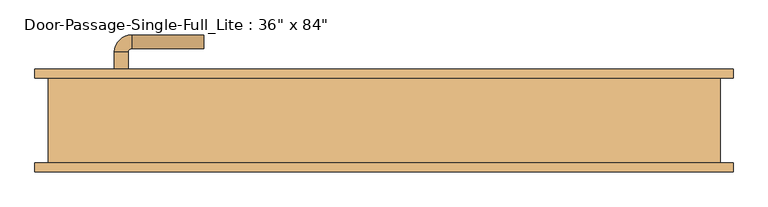
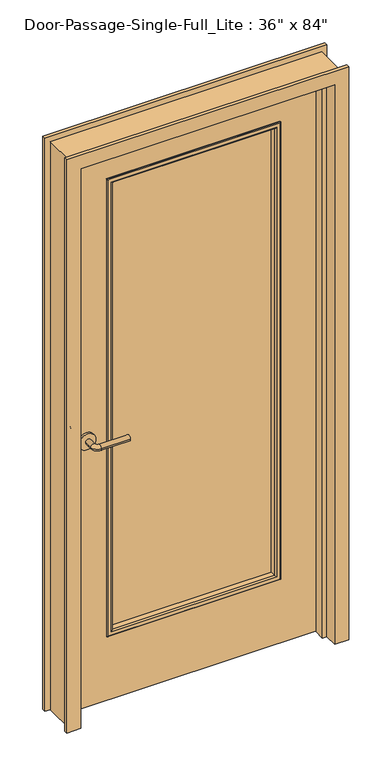
"""IFC4 building model written with IfcOpenShell, lengths in millimetres: door geometry."""

from ifc_helpers import new_model, si_unit, point, frame, frame_2d, origin, place, context, project, spatial, polyline, circle_curve, ellipse_curve, trimmed, segment, composite_curve, outline, extrude, faceted_brep, source, transform, mapped, element, save
from ifc_brep_helpers import plane_surface, cylinder_surface, revolved_surface, advanced_brep


def door_297712db(model_context):
    return source(origin(), model_context, "Body", "SolidModel", [
        advanced_brep(
        [(-392.190625, 15.8125, 1016.0), (-372.190625, 15.8125, 1016.0), (-372.190625, -14.1875, 1016.0), (-392.190625, -14.1875, 1016.0), (-367.190625, -19.1875, 1016.0), (-367.190625, -39.1875, 1016.0), (-262.190625, -39.1875, 1016.0), (-262.190625, -19.1875, 1016.0)],
        [
            (0, 1, circle_curve(frame((-382.190625, 15.8125, 1016.0), z_axis=(0.0, 1.0, 0.0), x_axis=(1.0, 0.0, 0.0)), 10.0)),
            (1, 0, circle_curve(frame((-382.190625, 15.8125, 1016.0), z_axis=(0.0, 1.0, 0.0), x_axis=(1.0, 0.0, 0.0)), 10.0)),
            (1, 2),
            (2, 3, circle_curve(frame((-382.190625, -14.1875, 1016.0), z_axis=(0.0, 1.0, 0.0), x_axis=(1.0, 0.0, 0.0)), 10.0)),
            (3, 0),
            (3, 2, circle_curve(frame((-382.190625, -14.1875, 1016.0), z_axis=(0.0, 1.0, 0.0), x_axis=(1.0, 0.0, 0.0)), 10.0)),
            (4, 5, circle_curve(frame((-367.190625, -29.1875, 1016.0), z_axis=(-1.0, 0.0, 0.0), x_axis=(0.0, 1.0, 0.0)), 10.0)),
            (5, 3, circle_curve(frame((-367.190625, -14.1875, 1016.0), z_axis=(0.0, 0.0, -1.0), x_axis=(-1.0, 0.0, 0.0)), 25.0)),
            (2, 4, circle_curve(frame((-367.190625, -14.1875, 1016.0), z_axis=(0.0, 0.0, 1.0), x_axis=(-1.0, 0.0, 0.0)), 5.0)),
            (5, 4, circle_curve(frame((-367.190625, -29.1875, 1016.0), z_axis=(-1.0, 0.0, 0.0), x_axis=(0.0, 1.0, 0.0)), 10.0)),
            (6, 7, circle_curve(frame((-262.190625, -29.1875, 1016.0), z_axis=(1.0, 0.0, 0.0), x_axis=(0.0, 1.0, 0.0)), 10.0)),
            (7, 6, circle_curve(frame((-262.190625, -29.1875, 1016.0), z_axis=(1.0, 0.0, 0.0), x_axis=(0.0, 1.0, 0.0)), 10.0)),
            (4, 7),
            (6, 5),
        ],
        [
            plane_surface(frame((-382.190625, 15.8125, 1016.0), z_axis=(0.0, 1.0, 0.0), x_axis=(0.0, 0.0, 1.0))),
            cylinder_surface(frame((-382.190625, 15.8125, 1016.0), z_axis=(0.0, 1.0, 0.0), x_axis=(1.0, 0.0, 0.0)), 10.0),
            revolved_surface(trimmed(ellipse_curve(frame((-382.190625, -14.1875, 1016.0), z_axis=(0.0, -1.0, 0.0), x_axis=(1.0, 0.0, 0.0)), 10.0, 10.0), [point((-392.190625, -14.1875, 1016.0))], [point((-372.190625, -14.1875, 1016.0))], True, "CARTESIAN"), (-367.190625, -14.1875, 1016.0), (0.0, 0.0, -1.0)),
            revolved_surface(trimmed(ellipse_curve(frame((-382.190625, -14.1875, 1016.0), z_axis=(0.0, -1.0, 0.0), x_axis=(1.0, 0.0, 0.0)), 10.0, 10.0), [point((-372.190625, -14.1875, 1016.0))], [point((-392.190625, -14.1875, 1016.0))], True, "CARTESIAN"), (-367.190625, -14.1875, 1016.0), (0.0, 0.0, -1.0)),
            plane_surface(frame((-262.190625, -29.1875, 1016.0), z_axis=(1.0, 0.0, 0.0), x_axis=(0.0, 0.0, 1.0))),
            cylinder_surface(frame((-367.190625, -29.1875, 1016.0), z_axis=(-1.0, 0.0, 0.0), x_axis=(0.0, 1.0, 0.0)), 10.0),
        ],
        [
            (0, [[1, 2]]),
            (1, [[3, 4, 5, -2]]),
            (1, [[-5, 6, -3, -1]]),
            (2, [[7, 8, -4, 9]]),
            (3, [[10, -9, -6, -8]]),
            (4, [[11, 12]]),
            (5, [[13, -11, 14, -7]]),
            (5, [[-14, -12, -13, -10]]),
        ],
    ),
        extrude(outline(composite_curve([segment(trimmed(circle_curve(frame_2d((1016.0, -384.690625)), 30.0), [point((1016.0, -414.690625))], [point((1016.0, -354.690625))], False, "CARTESIAN"), True, "CONTINUOUS"), segment(trimmed(circle_curve(frame_2d((1016.0, -384.690625)), 30.0), [point((1016.0, -354.690625))], [point((1016.0, -414.690625))], False, "CARTESIAN"), True, "CONTINUOUS")], self_intersect=False)), frame((0.0, 15.8125, 0.0), z_axis=(0.0, 1.0, 0.0), x_axis=(0.0, 0.0, 1.0)), (0.0, 0.0, 1.0), 8.0),
        advanced_brep(
        [(-392.190625, 76.2625, 1016.0), (-372.190625, 76.2625, 1016.0), (-392.190625, 106.2625, 1016.0), (-372.190625, 106.2625, 1016.0), (-367.190625, 111.2625, 1016.0), (-367.190625, 131.2625, 1016.0), (-262.190625, 131.2625, 1016.0), (-262.190625, 111.2625, 1016.0)],
        [
            (0, 1, circle_curve(frame((-382.190625, 76.2625, 1016.0), z_axis=(0.0, -1.0, 0.0), x_axis=(1.0, 0.0, 0.0)), 10.0)),
            (1, 0, circle_curve(frame((-382.190625, 76.2625, 1016.0), z_axis=(0.0, -1.0, 0.0), x_axis=(1.0, 0.0, 0.0)), 10.0)),
            (0, 2),
            (2, 3, circle_curve(frame((-382.190625, 106.2625, 1016.0), z_axis=(0.0, -1.0, 0.0), x_axis=(1.0, 0.0, 0.0)), 10.0)),
            (3, 1),
            (3, 2, circle_curve(frame((-382.190625, 106.2625, 1016.0), z_axis=(0.0, -1.0, 0.0), x_axis=(1.0, 0.0, 0.0)), 10.0)),
            (4, 3, circle_curve(frame((-367.190625, 106.2625, 1016.0), z_axis=(0.0, 0.0, 1.0), x_axis=(-1.0, 0.0, 0.0)), 5.0)),
            (2, 5, circle_curve(frame((-367.190625, 106.2625, 1016.0), z_axis=(0.0, 0.0, -1.0), x_axis=(-1.0, 0.0, 0.0)), 25.0)),
            (5, 4, circle_curve(frame((-367.190625, 121.2625, 1016.0), z_axis=(-1.0, 0.0, 0.0), x_axis=(0.0, -1.0, 0.0)), 10.0)),
            (4, 5, circle_curve(frame((-367.190625, 121.2625, 1016.0), z_axis=(-1.0, 0.0, 0.0), x_axis=(0.0, -1.0, 0.0)), 10.0)),
            (6, 7, circle_curve(frame((-262.190625, 121.2625, 1016.0), z_axis=(1.0, 0.0, 0.0), x_axis=(0.0, -1.0, 0.0)), 10.0)),
            (7, 6, circle_curve(frame((-262.190625, 121.2625, 1016.0), z_axis=(1.0, 0.0, 0.0), x_axis=(0.0, -1.0, 0.0)), 10.0)),
            (5, 6),
            (7, 4),
        ],
        [
            plane_surface(frame((-382.190625, 76.2625, 1016.0), z_axis=(0.0, -1.0, 0.0), x_axis=(0.0, 0.0, 1.0))),
            cylinder_surface(frame((-382.190625, 76.2625, 1016.0), z_axis=(0.0, -1.0, 0.0), x_axis=(1.0, 0.0, 0.0)), 10.0),
            revolved_surface(trimmed(ellipse_curve(frame((-382.190625, 106.2625, 1016.0), z_axis=(0.0, -1.0, 0.0), x_axis=(1.0, 0.0, 0.0)), 10.0, 10.0), [point((-392.190625, 106.2625, 1016.0))], [point((-372.190625, 106.2625, 1016.0))], True, "CARTESIAN"), (-367.190625, 106.2625, 1016.0), (0.0, 0.0, -1.0)),
            revolved_surface(trimmed(ellipse_curve(frame((-382.190625, 106.2625, 1016.0), z_axis=(0.0, -1.0, 0.0), x_axis=(1.0, 0.0, 0.0)), 10.0, 10.0), [point((-372.190625, 106.2625, 1016.0))], [point((-392.190625, 106.2625, 1016.0))], True, "CARTESIAN"), (-367.190625, 106.2625, 1016.0), (0.0, 0.0, -1.0)),
            plane_surface(frame((-262.190625, 121.2625, 1016.0), z_axis=(1.0, 0.0, 0.0), x_axis=(0.0, 0.0, 1.0))),
            cylinder_surface(frame((-367.190625, 121.2625, 1016.0), z_axis=(-1.0, 0.0, 0.0), x_axis=(0.0, -1.0, 0.0)), 10.0),
        ],
        [
            (0, [[1, 2]]),
            (1, [[-1, 3, 4, 5]]),
            (1, [[-2, -5, 6, -3]]),
            (2, [[7, -4, 8, 9]]),
            (3, [[-8, -6, -7, 10]]),
            (4, [[11, 12]]),
            (5, [[-9, 13, -12, 14]]),
            (5, [[-10, -14, -11, -13]]),
        ],
    ),
        extrude(outline(composite_curve([segment(trimmed(circle_curve(frame_2d((1016.0, -384.690625)), 30.0), [point((1016.0, -414.690625))], [point((1016.0, -354.690625))], False, "CARTESIAN"), True, "CONTINUOUS"), segment(trimmed(circle_curve(frame_2d((1016.0, -384.690625)), 30.0), [point((1016.0, -354.690625))], [point((1016.0, -414.690625))], False, "CARTESIAN"), True, "CONTINUOUS")], self_intersect=False)), frame((0.0, 68.2625, 0.0), z_axis=(0.0, 1.0, 0.0), x_axis=(0.0, 0.0, 1.0)), (0.0, 0.0, 1.0), 8.0),
        extrude(outline(polyline([(304.8, 42.8625), (-304.8, 42.8625), (-304.8, 49.2125), (304.8, 49.2125), (304.8, 42.8625)])), frame((0.0, 0.0, 254.0), z_axis=(0.0, 0.0, 1.0), x_axis=(1.0, 0.0, 0.0)), (0.0, 0.0, 1.0), 1727.2),
        faceted_brep([(457.2, 80.9625, 0.0), (508.0, 80.9625, 0.0), (508.0, 68.2625, 0.0), (488.95, 68.2625, 0.0), (488.95, -55.5625, 0.0), (508.0, -55.5625, 0.0), (508.0, -68.2625, 0.0), (457.2, -68.2625, 0.0), (457.2, -19.05, 0.0), (441.325, -19.05, 0.0), (441.325, 19.05, 0.0), (457.2, 19.05, 0.0), (457.2, 80.9625, 2133.6), (-457.2, 80.9625, 2133.6), (-457.2, 80.9625, 0.0), (-508.0, 80.9625, 0.0), (-508.0, 80.9625, 2184.4), (508.0, 80.9625, 2184.4), (508.0, 68.2625, 2184.4), (-508.0, 68.2625, 2184.4), (-508.0, 68.2625, 0.0), (-488.95, 68.2625, 0.0), (-488.95, 68.2625, 2165.35), (488.95, 68.2625, 2165.35), (488.95, -55.5625, 2165.35), (-488.95, -55.5625, 2165.35), (-488.95, -55.5625, 0.0), (-508.0, -55.5625, 0.0), (-508.0, -55.5625, 2184.4), (508.0, -55.5625, 2184.4), (508.0, -68.2625, 2184.4), (-508.0, -68.2625, 2184.4), (-508.0, -68.2625, 0.0), (-457.2, -68.2625, 0.0), (-457.2, -68.2625, 2133.6), (457.2, -68.2625, 2133.6), (457.2, -19.05, 2133.6), (-457.2, -19.05, 2133.6), (-457.2, -19.05, 0.0), (-441.325, -19.05, 0.0), (-441.325, -19.05, 2117.725), (441.325, -19.05, 2117.725), (441.325, 19.05, 2117.725), (-441.325, 19.05, 2117.725), (-441.325, 19.05, 0.0), (-457.2, 19.05, 0.0), (-457.2, 19.05, 2133.6), (457.2, 19.05, 2133.6)], [[[0, 1, 2, 3, 4, 5, 6, 7, 8, 9, 10, 11]], [[1, 0, 12, 13, 14, 15, 16, 17]], [[2, 1, 17, 18]], [[3, 2, 18, 19, 20, 21, 22, 23]], [[4, 3, 23, 24]], [[5, 4, 24, 25, 26, 27, 28, 29]], [[6, 5, 29, 30]], [[7, 6, 30, 31, 32, 33, 34, 35]], [[8, 7, 35, 36]], [[9, 8, 36, 37, 38, 39, 40, 41]], [[10, 9, 41, 42]], [[11, 10, 42, 43, 44, 45, 46, 47]], [[0, 11, 47, 12]], [[18, 17, 16, 19]], [[24, 23, 22, 25]], [[30, 29, 28, 31]], [[36, 35, 34, 37]], [[42, 41, 40, 43]], [[12, 47, 46, 13]], [[14, 45, 44, 39, 38, 33, 32, 27, 26, 21, 20, 15]], [[19, 16, 15, 20]], [[25, 22, 21, 26]], [[31, 28, 27, 32]], [[37, 34, 33, 38]], [[43, 40, 39, 44]], [[13, 46, 45, 14]]]),
        extrude(outline(polyline([(2133.6, -457.2), (0.0, -457.2), (0.0, 457.2), (2133.6, 457.2), (2133.6, -457.2)]), holes=[polyline([(1981.2, -304.8), (1981.2, 304.8), (254.0, 304.8), (254.0, -304.8), (1981.2, -304.8)])]), frame((0.0, 23.8125, 0.0), z_axis=(0.0, 1.0, 0.0), x_axis=(0.0, 0.0, 1.0)), (0.0, 0.0, 1.0), 44.45),
        advanced_brep(
        [(-304.8, 49.2125, 1981.2), (-304.8, 68.2625, 1981.2), (-304.8, 68.2625, 254.0), (-304.8, 49.2125, 254.0), (-292.8, 69.2625, 1969.2), (-292.8, 49.2125, 1969.2), (-292.8, 49.2125, 266.0), (-292.8, 69.2625, 266.0), (-297.8, 74.2625, 1974.2), (-297.8, 74.2625, 261.0), (-312.8, 72.2625, 1989.2), (-310.8, 74.2625, 1987.2), (-310.8, 74.2625, 248.0), (-312.8, 72.2625, 246.0), (-312.8, 68.2625, 1989.2), (-312.8, 68.2625, 246.0), (304.8, 68.2625, 254.0), (304.8, 49.2125, 254.0), (292.8, 49.2125, 266.0), (292.8, 69.2625, 266.0), (297.8, 74.2625, 261.0), (310.8, 74.2625, 248.0), (312.8, 72.2625, 246.0), (312.8, 68.2625, 246.0), (304.8, 68.2625, 1981.2), (304.8, 49.2125, 1981.2), (292.8, 49.2125, 1969.2), (292.8, 69.2625, 1969.2), (297.8, 74.2625, 1974.2), (310.8, 74.2625, 1987.2), (312.8, 72.2625, 1989.2), (312.8, 68.2625, 1989.2)],
        [
            (0, 1),
            (1, 2),
            (2, 3),
            (3, 0),
            (4, 5),
            (5, 6),
            (6, 7),
            (7, 4),
            (8, 4, ellipse_curve(frame((-297.8, 69.2625, 1974.2), z_axis=(-0.7071067811865475, 0.0, -0.7071067811865475), x_axis=(-0.7071067811865474, 0.0, 0.7071067811865476)), 7.0710678, 5.0)),
            (7, 9, ellipse_curve(frame((-297.8, 69.2625, 261.0), z_axis=(-0.7071067811865475, 0.0, 0.7071067811865475), x_axis=(0.7071067811865474, 0.0, 0.7071067811865476)), 7.0710678, 5.0)),
            (9, 8),
            (10, 11, ellipse_curve(frame((-310.8, 72.2625, 1987.2), z_axis=(-0.7071067811865475, 0.0, -0.7071067811865475), x_axis=(-0.7071067811865474, 0.0, 0.7071067811865476)), 2.8284271, 2.0)),
            (11, 12),
            (12, 13, ellipse_curve(frame((-310.8, 72.2625, 248.0), z_axis=(-0.7071067811865475, 0.0, 0.7071067811865475), x_axis=(0.7071067811865474, 0.0, 0.7071067811865476)), 2.8284271, 2.0)),
            (13, 10),
            (14, 10),
            (13, 15),
            (15, 14),
            (2, 16),
            (16, 17),
            (17, 3),
            (6, 18),
            (18, 19),
            (19, 7),
            (19, 20, ellipse_curve(frame((297.8, 69.2625, 261.0), z_axis=(-0.7071067811865475, 0.0, -0.7071067811865475), x_axis=(-0.7071067811865476, 0.0, 0.7071067811865474)), 7.0710678, 5.0)),
            (20, 9),
            (12, 21),
            (21, 22, ellipse_curve(frame((310.8, 72.2625, 248.0), z_axis=(-0.7071067811865475, 0.0, -0.7071067811865475), x_axis=(-0.7071067811865476, 0.0, 0.7071067811865474)), 2.8284271, 2.0)),
            (22, 13),
            (22, 23),
            (23, 15),
            (16, 24),
            (24, 25),
            (25, 17),
            (18, 26),
            (26, 27),
            (27, 19),
            (27, 28, ellipse_curve(frame((297.8, 69.2625, 1974.2), z_axis=(0.7071067811865475, 0.0, -0.7071067811865475), x_axis=(-0.7071067811865474, 0.0, -0.7071067811865476)), 7.0710678, 5.0)),
            (28, 20),
            (21, 29),
            (29, 30, ellipse_curve(frame((310.8, 72.2625, 1987.2), z_axis=(0.7071067811865475, 0.0, -0.7071067811865475), x_axis=(-0.7071067811865474, 0.0, -0.7071067811865476)), 2.8284271, 2.0)),
            (30, 22),
            (30, 31),
            (31, 23),
            (31, 14),
            (1, 24),
            (0, 25),
            (5, 26),
            (4, 27),
            (8, 28),
            (11, 29),
            (10, 30),
        ],
        [
            plane_surface(frame((-304.8, 68.2625, 1981.2), z_axis=(-1.0, 0.0, 0.0), x_axis=(0.0, 0.0, -1.0))),
            plane_surface(frame((-292.8, 49.2125, 1969.2), z_axis=(1.0, 0.0, 0.0), x_axis=(0.0, 0.0, -1.0))),
            cylinder_surface(frame((-297.8, 69.2625, 1981.2), z_axis=(0.0, 0.0, 1.0), x_axis=(-1.0, 0.0, 0.0)), 5.0),
            cylinder_surface(frame((-310.8, 72.2625, 1981.2), z_axis=(0.0, 0.0, 1.0), x_axis=(-1.0, 0.0, 0.0)), 2.0),
            plane_surface(frame((-312.8, 72.2625, 1989.2), z_axis=(-1.0, 0.0, 0.0), x_axis=(0.0, 0.0, -1.0))),
            plane_surface(frame((-304.8, 68.2625, 254.0), z_axis=(0.0, 0.0, -1.0), x_axis=(1.0, 0.0, 0.0))),
            plane_surface(frame((-292.8, 49.2125, 266.0), z_axis=(0.0, 0.0, 1.0), x_axis=(1.0, 0.0, 0.0))),
            cylinder_surface(frame((-304.8, 69.2625, 261.0), z_axis=(-1.0, 0.0, 0.0), x_axis=(0.0, 0.0, -1.0)), 5.0),
            cylinder_surface(frame((-304.8, 72.2625, 248.0), z_axis=(-1.0, 0.0, 0.0), x_axis=(0.0, 0.0, -1.0)), 2.0),
            plane_surface(frame((-312.8, 72.2625, 246.0), z_axis=(0.0, 0.0, -1.0), x_axis=(1.0, 0.0, 0.0))),
            plane_surface(frame((304.8, 68.2625, 254.0), z_axis=(1.0, 0.0, 0.0), x_axis=(0.0, 0.0, 1.0))),
            plane_surface(frame((292.8, 49.2125, 266.0), z_axis=(-1.0, 0.0, 0.0), x_axis=(0.0, 0.0, 1.0))),
            cylinder_surface(frame((297.8, 69.2625, 254.0), z_axis=(0.0, 0.0, -1.0), x_axis=(1.0, 0.0, 0.0)), 5.0),
            cylinder_surface(frame((310.8, 72.2625, 254.0), z_axis=(0.0, 0.0, -1.0), x_axis=(1.0, 0.0, 0.0)), 2.0),
            plane_surface(frame((312.8, 72.2625, 246.0), z_axis=(1.0, 0.0, 0.0), x_axis=(0.0, 0.0, 1.0))),
            plane_surface(frame((312.8, 68.2625, 1989.2), z_axis=(0.0, -1.0, 0.0), x_axis=(-1.0, 0.0, 0.0))),
            plane_surface(frame((304.8, 68.2625, 1981.2), z_axis=(0.0, 0.0, 1.0), x_axis=(-1.0, 0.0, 0.0))),
            plane_surface(frame((304.8, 49.2125, 1981.2), z_axis=(0.0, -1.0, 0.0), x_axis=(-1.0, 0.0, 0.0))),
            plane_surface(frame((292.8, 49.2125, 1969.2), z_axis=(0.0, 0.0, -1.0), x_axis=(-1.0, 0.0, 0.0))),
            cylinder_surface(frame((304.8, 69.2625, 1974.2), z_axis=(1.0, 0.0, 0.0), x_axis=(0.0, 0.0, 1.0)), 5.0),
            plane_surface(frame((297.8, 74.2625, 1974.2), z_axis=(0.0, 1.0, 0.0), x_axis=(-1.0, 0.0, 0.0))),
            cylinder_surface(frame((304.8, 72.2625, 1987.2), z_axis=(1.0, 0.0, 0.0), x_axis=(0.0, 0.0, 1.0)), 2.0),
            plane_surface(frame((312.8, 72.2625, 1989.2), z_axis=(0.0, 0.0, 1.0), x_axis=(-1.0, 0.0, 0.0))),
        ],
        [
            (0, [[1, 2, 3, 4]]),
            (1, [[5, 6, 7, 8]]),
            (2, [[9, -8, 10, 11]]),
            (3, [[12, 13, 14, 15]]),
            (4, [[16, -15, 17, 18]]),
            (5, [[-3, 19, 20, 21]]),
            (6, [[-7, 22, 23, 24]]),
            (7, [[-10, -24, 25, 26]]),
            (8, [[-14, 27, 28, 29]]),
            (9, [[-17, -29, 30, 31]]),
            (10, [[-20, 32, 33, 34]]),
            (11, [[-23, 35, 36, 37]]),
            (12, [[-25, -37, 38, 39]]),
            (13, [[-28, 40, 41, 42]]),
            (14, [[-30, -42, 43, 44]]),
            (15, [[-31, -44, 45, -18], [46, -32, -19, -2]]),
            (16, [[-33, -46, -1, 47]]),
            (17, [[-21, -34, -47, -4], [48, -35, -22, -6]]),
            (18, [[-36, -48, -5, 49]]),
            (19, [[-38, -49, -9, 50]]),
            (20, [[51, -40, -27, -13], [-26, -39, -50, -11]]),
            (21, [[-41, -51, -12, 52]]),
            (22, [[-43, -52, -16, -45]]),
        ],
    ),
        advanced_brep(
        [(-304.8, 42.8625, 254.0), (-304.8, 23.8125, 254.0), (-304.8, 23.8125, 1981.2), (-304.8, 42.8625, 1981.2), (-292.8, 22.8125, 266.0), (-292.8, 42.8625, 266.0), (-292.8, 42.8625, 1969.2), (-292.8, 22.8125, 1969.2), (-297.8, 17.8125, 261.0), (-297.8, 17.8125, 1974.2), (-312.8, 19.8125, 246.0), (-310.8, 17.8125, 248.0), (-310.8, 17.8125, 1987.2), (-312.8, 19.8125, 1989.2), (-312.8, 23.8125, 246.0), (-312.8, 23.8125, 1989.2), (304.8, 23.8125, 1981.2), (304.8, 42.8625, 1981.2), (292.8, 42.8625, 1969.2), (292.8, 22.8125, 1969.2), (297.8, 17.8125, 1974.2), (310.8, 17.8125, 1987.2), (312.8, 19.8125, 1989.2), (312.8, 23.8125, 1989.2), (304.8, 23.8125, 254.0), (304.8, 42.8625, 254.0), (292.8, 42.8625, 266.0), (292.8, 22.8125, 266.0), (297.8, 17.8125, 261.0), (310.8, 17.8125, 248.0), (312.8, 19.8125, 246.0), (312.8, 23.8125, 246.0)],
        [
            (0, 1),
            (1, 2),
            (2, 3),
            (3, 0),
            (4, 5),
            (5, 6),
            (6, 7),
            (7, 4),
            (8, 4, ellipse_curve(frame((-297.8, 22.8125, 261.0), z_axis=(-0.7071067811865475, 0.0, 0.7071067811865475), x_axis=(-0.7071067811865474, 0.0, -0.7071067811865476)), 7.0710678, 5.0)),
            (7, 9, ellipse_curve(frame((-297.8, 22.8125, 1974.2), z_axis=(-0.7071067811865475, 0.0, -0.7071067811865475), x_axis=(0.7071067811865474, 0.0, -0.7071067811865476)), 7.0710678, 5.0)),
            (9, 8),
            (10, 11, ellipse_curve(frame((-310.8, 19.8125, 248.0), z_axis=(-0.7071067811865475, 0.0, 0.7071067811865475), x_axis=(-0.7071067811865474, 0.0, -0.7071067811865476)), 2.8284271, 2.0)),
            (11, 12),
            (12, 13, ellipse_curve(frame((-310.8, 19.8125, 1987.2), z_axis=(-0.7071067811865475, 0.0, -0.7071067811865475), x_axis=(0.7071067811865474, 0.0, -0.7071067811865476)), 2.8284271, 2.0)),
            (13, 10),
            (14, 10),
            (13, 15),
            (15, 14),
            (2, 16),
            (16, 17),
            (17, 3),
            (6, 18),
            (18, 19),
            (19, 7),
            (19, 20, ellipse_curve(frame((297.8, 22.8125, 1974.2), z_axis=(-0.7071067811865475, 0.0, 0.7071067811865475), x_axis=(-0.7071067811865476, 0.0, -0.7071067811865474)), 7.0710678, 5.0)),
            (20, 9),
            (12, 21),
            (21, 22, ellipse_curve(frame((310.8, 19.8125, 1987.2), z_axis=(-0.7071067811865475, 0.0, 0.7071067811865475), x_axis=(-0.7071067811865476, 0.0, -0.7071067811865474)), 2.8284271, 2.0)),
            (22, 13),
            (22, 23),
            (23, 15),
            (16, 24),
            (24, 25),
            (25, 17),
            (18, 26),
            (26, 27),
            (27, 19),
            (27, 28, ellipse_curve(frame((297.8, 22.8125, 261.0), z_axis=(0.7071067811865475, 0.0, 0.7071067811865475), x_axis=(-0.7071067811865474, 0.0, 0.7071067811865476)), 7.0710678, 5.0)),
            (28, 20),
            (21, 29),
            (29, 30, ellipse_curve(frame((310.8, 19.8125, 248.0), z_axis=(0.7071067811865475, 0.0, 0.7071067811865475), x_axis=(-0.7071067811865474, 0.0, 0.7071067811865476)), 2.8284271, 2.0)),
            (30, 22),
            (30, 31),
            (31, 23),
            (31, 14),
            (1, 24),
            (0, 25),
            (5, 26),
            (4, 27),
            (8, 28),
            (11, 29),
            (10, 30),
        ],
        [
            plane_surface(frame((-304.8, 23.8125, 254.0), z_axis=(-1.0, 0.0, 0.0), x_axis=(0.0, 0.0, 1.0))),
            plane_surface(frame((-292.8, 42.8625, 266.0), z_axis=(1.0, 0.0, 0.0), x_axis=(0.0, 0.0, 1.0))),
            cylinder_surface(frame((-297.8, 22.8125, 254.0), z_axis=(0.0, 0.0, -1.0), x_axis=(-1.0, 0.0, 0.0)), 5.0),
            cylinder_surface(frame((-310.8, 19.8125, 254.0), z_axis=(0.0, 0.0, -1.0), x_axis=(-1.0, 0.0, 0.0)), 2.0),
            plane_surface(frame((-312.8, 19.8125, 246.0), z_axis=(-1.0, 0.0, 0.0), x_axis=(0.0, 0.0, 1.0))),
            plane_surface(frame((-304.8, 23.8125, 1981.2), z_axis=(0.0, 0.0, 1.0), x_axis=(1.0, 0.0, 0.0))),
            plane_surface(frame((-292.8, 42.8625, 1969.2), z_axis=(0.0, 0.0, -1.0), x_axis=(1.0, 0.0, 0.0))),
            cylinder_surface(frame((-304.8, 22.8125, 1974.2), z_axis=(-1.0, 0.0, 0.0), x_axis=(0.0, 0.0, 1.0)), 5.0),
            cylinder_surface(frame((-304.8, 19.8125, 1987.2), z_axis=(-1.0, 0.0, 0.0), x_axis=(0.0, 0.0, 1.0)), 2.0),
            plane_surface(frame((-312.8, 19.8125, 1989.2), z_axis=(0.0, 0.0, 1.0), x_axis=(1.0, 0.0, 0.0))),
            plane_surface(frame((304.8, 23.8125, 1981.2), z_axis=(1.0, 0.0, 0.0), x_axis=(0.0, 0.0, -1.0))),
            plane_surface(frame((292.8, 42.8625, 1969.2), z_axis=(-1.0, 0.0, 0.0), x_axis=(0.0, 0.0, -1.0))),
            cylinder_surface(frame((297.8, 22.8125, 1981.2), z_axis=(0.0, 0.0, 1.0), x_axis=(1.0, 0.0, 0.0)), 5.0),
            cylinder_surface(frame((310.8, 19.8125, 1981.2), z_axis=(0.0, 0.0, 1.0), x_axis=(1.0, 0.0, 0.0)), 2.0),
            plane_surface(frame((312.8, 19.8125, 1989.2), z_axis=(1.0, 0.0, 0.0), x_axis=(0.0, 0.0, -1.0))),
            plane_surface(frame((312.8, 23.8125, 246.0), z_axis=(0.0, 1.0, 0.0), x_axis=(-1.0, 0.0, 0.0))),
            plane_surface(frame((304.8, 23.8125, 254.0), z_axis=(0.0, 0.0, -1.0), x_axis=(-1.0, 0.0, 0.0))),
            plane_surface(frame((304.8, 42.8625, 254.0), z_axis=(0.0, 1.0, 0.0), x_axis=(-1.0, 0.0, 0.0))),
            plane_surface(frame((292.8, 42.8625, 266.0), z_axis=(0.0, 0.0, 1.0), x_axis=(-1.0, 0.0, 0.0))),
            cylinder_surface(frame((304.8, 22.8125, 261.0), z_axis=(1.0, 0.0, 0.0), x_axis=(0.0, 0.0, -1.0)), 5.0),
            plane_surface(frame((297.8, 17.8125, 261.0), z_axis=(0.0, -1.0, 0.0), x_axis=(-1.0, 0.0, 0.0))),
            cylinder_surface(frame((304.8, 19.8125, 248.0), z_axis=(1.0, 0.0, 0.0), x_axis=(0.0, 0.0, -1.0)), 2.0),
            plane_surface(frame((312.8, 19.8125, 246.0), z_axis=(0.0, 0.0, -1.0), x_axis=(-1.0, 0.0, 0.0))),
        ],
        [
            (0, [[1, 2, 3, 4]]),
            (1, [[5, 6, 7, 8]]),
            (2, [[9, -8, 10, 11]]),
            (3, [[12, 13, 14, 15]]),
            (4, [[16, -15, 17, 18]]),
            (5, [[-3, 19, 20, 21]]),
            (6, [[-7, 22, 23, 24]]),
            (7, [[-10, -24, 25, 26]]),
            (8, [[-14, 27, 28, 29]]),
            (9, [[-17, -29, 30, 31]]),
            (10, [[-20, 32, 33, 34]]),
            (11, [[-23, 35, 36, 37]]),
            (12, [[-25, -37, 38, 39]]),
            (13, [[-28, 40, 41, 42]]),
            (14, [[-30, -42, 43, 44]]),
            (15, [[-31, -44, 45, -18], [46, -32, -19, -2]]),
            (16, [[-33, -46, -1, 47]]),
            (17, [[-21, -34, -47, -4], [48, -35, -22, -6]]),
            (18, [[-36, -48, -5, 49]]),
            (19, [[-38, -49, -9, 50]]),
            (20, [[51, -40, -27, -13], [-26, -39, -50, -11]]),
            (21, [[-41, -51, -12, 52]]),
            (22, [[-43, -52, -16, -45]]),
        ],
    ),
    ])


if __name__ == "__main__":
    model = new_model("IFC4")
    model_context = context("Model", 3, world=origin())
    ifc_project = project(units=[si_unit("LENGTHUNIT", "METRE", prefix="MILLI")], contexts=[model_context])
    site = spatial("IfcSite", under=ifc_project)
    building = spatial("IfcBuilding", under=site)
    placement = place(None, origin())
    door_shape = door_297712db(model_context)
    element("IfcDoor", 1, ObjectType="Door-Passage-Single-Full_Lite : 36\" x 84\"", at=placement, inside=building, context=model_context, shape_type="MappedRepresentation", body=[
        mapped(door_shape, transform((0.0, 0.0, 0.0), x_axis=(1.0, 0.0, 0.0), y_axis=(0.0, 1.0, 0.0), z_axis=(0.0, 0.0, 1.0))),
    ])
    save(model, "model.ifc")

# Revit data of these elements
# Type "Door-Passage-Single-Full_Lite : 36\" x 84\""
#   Type Mark = "33"
#   Assembly Code = "B2030100"
#   Analytic Construction = "Wooden"
#   Thickness = 0' - 1 3/4"
#   Thermal Resistance (R) = 2.5876 (h·ft²·°F)/BTU
#   Swing Angle [instance default] = 90.00°
#   Strike Height = 3' - 4"
#   Rough Width [instance default] = 3' - 4"
#   Rough Height [instance default] = 7' - 4"
#   MF Opening Height [instance default] = 0' - 4"
#   MF Opening Width [instance default] = 0' - 4"
#   Inset Calculate [instance default] = 0' - 4"
#   Masonry Inset [instance default] = 0' - 1"
#   Height = 7' - 0"
#   Width = 3' - 0"
#   Heat Transfer Coefficient (U) = 0.3865 BTU/(h·ft²·°F)
#   Masonry Frame Depth = 0' - 5 3/4"
#   Masonry Frame [instance default] = yes
#   Function = 1
#   Dry Wall Frame [instance default] = no
#   Panel Material = Wood - Birch
#   Glazing = Glass
#   Glass Stop Material = Metal - Paint Finish - Grey
#   Frame Material = Metal - Paint Finish - Grey
#   Door Handle Material = Aluminum
#   Visual Light Transmittance = 0
#   Solar Heat Gain Coefficient = 0
#   Wall Closure = (empty or 0)
# Element 1 (IfcDoor, "Door-Passage-Single-Full_Lite : 36\" x 84\"")
#   Rough Width = 3' - 2 1/2"
#   Rough Height = 7' - 1 1/4"
#   MF Opening Height = 0' - 1 1/4"
#   MF Opening Width = 0' - 2 1/2"
#   Inset Calculate = 0' - 3"
#   Masonry Frame = no
#   Dry Wall Frame = yes
#   Materials on its faces: "Metal - Paint Finish - Grey", "Aluminum", "Wood - Birch", "Glass"
# Materials
#   "Wood - Birch": class "Wood", colour RGB 166 116 52, transparency 0, Cost = 0
#   "Glass": class "Glass", colour RGB 0 128 192, transparency 0.75, Description = "Soda Lime Glass", Cost = 0
#   "Metal - Paint Finish - Grey": class "Paint", colour RGB 104 104 104, transparency 0, Cost = 0
#   "Aluminum": class "Metal", colour RGB 247 247 247, transparency 0, Description = "Aluminum 6061", Cost = 0
